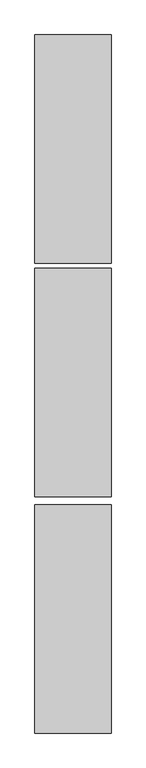
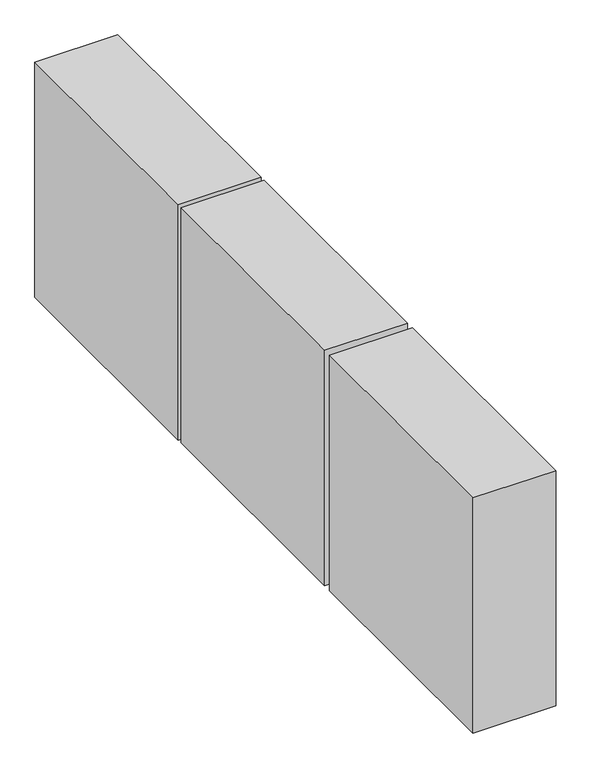
"""IFC4 building model written with IfcOpenShell, lengths in millimetres: furniture geometry, Metalic shelf : Metalic shelf."""

from ifc_helpers import new_model, si_unit, origin, origin_with_axes, place, context, project, spatial, polyline, outline, extrude, source, transform, mapped, element, save


def furniture_fd3c48cc(model_context):
    return source(origin(), model_context, "Body", "SweptSolid", [
        extrude(outline(polyline([(24289.5370052, 4217.6615366), (23984.7370052, 4217.6615366), (23984.7370052, 5132.0615366), (24289.5370052, 5132.0615366), (24289.5370052, 4217.6615366)])), origin_with_axes(), (0.0, 0.0, 1.0), 914.4),
        extrude(outline(polyline([(24289.5370052, 3271.5115366), (23984.7370052, 3271.5115366), (23984.7370052, 4185.9115366), (24289.5370052, 4185.9115366), (24289.5370052, 3271.5115366)])), origin_with_axes(), (0.0, 0.0, 1.0), 914.4),
        extrude(outline(polyline([(24289.5370052, 5151.1115366), (23984.7370052, 5151.1115366), (23984.7370052, 6065.5115366), (24289.5370052, 6065.5115366), (24289.5370052, 5151.1115366)])), origin_with_axes(), (0.0, 0.0, 1.0), 914.4),
    ])


if __name__ == "__main__":
    model = new_model("IFC4")
    model_context = context("Model", 3, world=origin())
    ifc_project = project(units=[si_unit("LENGTHUNIT", "METRE", prefix="MILLI")], contexts=[model_context])
    site = spatial("IfcSite", under=ifc_project)
    building = spatial("IfcBuilding", under=site)
    placement = place(None, origin())
    furniture_shape = furniture_fd3c48cc(model_context)
    element("IfcFurniture", 1, ObjectType="Metalic shelf : Metalic shelf", at=placement, inside=building, context=model_context, shape_type="MappedRepresentation", body=[
        mapped(furniture_shape, transform((0.0, 0.0, 0.0), x_axis=(1.0, 0.0, 0.0), y_axis=(0.0, 1.0, 0.0), z_axis=(0.0, 0.0, 1.0))),
    ])
    save(model, "model.ifc")
